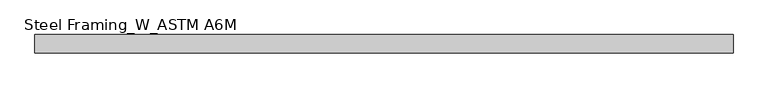
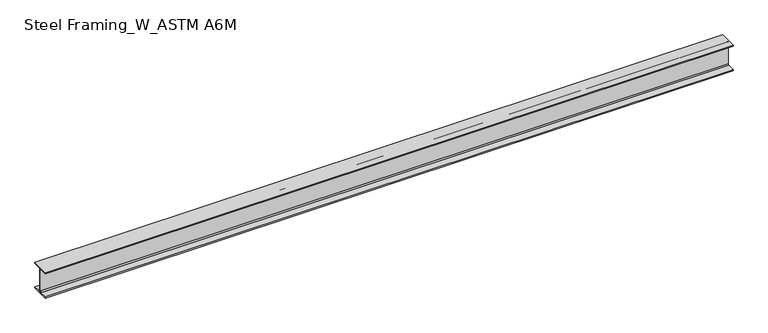
"""IFC4 building model written with IfcOpenShell, lengths in millimetres: beam geometry, Steel Framing_W_ASTM A6M : H_SB_AR_S02_W310x60_B5."""

import ifcopenshell
import ifcopenshell.guid

model = None  # the IFC model being written
_history = None  # IfcOwnerHistory: only IFC2X3 demands one
_inside = {}  # id of a spatial element -> (the spatial element, [elements in it])
_under = {}  # id of a project, library or spatial element -> (it, [spatial elements below it])
_declared = {}  # id of a project -> (the project, [libraries it declares])
_typed = {}  # id of a type object -> (the type object, [elements of that type])
_made_of = {}  # id of a material, layer set ... -> (it, [elements and type objects made of it])


def new_model(schema):
    """Start an empty IFC model of exactly this schema.

    Asked for "IFC4X3", IfcOpenShell would pick the latest addendum, in which some entities
    have other attributes; the version numbers below select the first issue.
    IFC2X3 requires an IfcOwnerHistory on every rooted entity: one is made here for all.
    """
    global model, _history
    if schema == "IFC4X3":
        model = ifcopenshell.file(schema_version=(4, 3, 0, 0))
    else:
        model = ifcopenshell.file(schema=schema)
    _inside.clear()
    _under.clear()
    _declared.clear()
    _typed.clear()
    _made_of.clear()
    _history = None
    if model.schema == "IFC2X3":
        org = make("IfcOrganization", Name="unknown")
        user = make(
            "IfcPersonAndOrganization",
            ThePerson=make("IfcPerson", FamilyName="unknown"),
            TheOrganization=org,
        )
        app = make(
            "IfcApplication",
            ApplicationDeveloper=org,
            Version="unknown",
            ApplicationFullName="unknown",
            ApplicationIdentifier="unknown",
        )
        _history = make(
            "IfcOwnerHistory",
            OwningUser=user,
            OwningApplication=app,
            ChangeAction="ADDED",
            CreationDate=0,
        )
    return model


def make(cls, **values):
    """One entity of the class cls with the attributes given. An attribute that is None is left unset."""
    return model.create_entity(
        cls, **{name: value for name, value in values.items() if value is not None}
    )


def rooted(cls, **values):
    """An entity with a GlobalId (a new one), such as an element, a storey or a relation."""
    return make(cls, GlobalId=ifcopenshell.guid.new(), OwnerHistory=_history, **values)


def si_unit(unit_type, name, prefix=None):
    """IfcSIUnit, for example si_unit("LENGTHUNIT", "METRE", prefix="MILLI")."""
    return make("IfcSIUnit", UnitType=unit_type, Prefix=prefix, Name=name)


def assignment(units):
    """IfcUnitAssignment: the units of a project."""
    return None if units is None else make("IfcUnitAssignment", Units=units)


def point(xyz):
    """IfcCartesianPoint."""
    return None if xyz is None else make("IfcCartesianPoint", Coordinates=xyz)


def direction(xyz):
    """IfcDirection."""
    return None if xyz is None else make("IfcDirection", DirectionRatios=xyz)


def frame(location, z_axis=None, x_axis=None):
    """IfcAxis2Placement3D, a coordinate frame: its origin and axes. An axis left out is left unset."""
    return make(
        "IfcAxis2Placement3D",
        Location=point(location),
        Axis=direction(z_axis),
        RefDirection=direction(x_axis),
    )


def frame_2d(location, x_axis=None):
    """IfcAxis2Placement2D, a coordinate frame in the plane: its origin and x axis."""
    return make(
        "IfcAxis2Placement2D", Location=point(location), RefDirection=direction(x_axis)
    )


def origin():
    """The frame at (0, 0, 0) with its axes left unset."""
    return frame((0.0, 0.0, 0.0))


def place(relative_to, where):
    """IfcLocalPlacement: puts the frame where relative to a parent placement (None: the world)."""
    return make(
        "IfcLocalPlacement", PlacementRelTo=relative_to, RelativePlacement=where
    )


def context(
    kind, dimensions, precision=None, world=None, true_north=None, identifier=None
):
    """IfcGeometricRepresentationContext, for example the 3D "Model" context."""
    return make(
        "IfcGeometricRepresentationContext",
        ContextIdentifier=identifier,
        ContextType=kind,
        CoordinateSpaceDimension=dimensions,
        Precision=precision,
        WorldCoordinateSystem=world,
        TrueNorth=true_north,
    )


def project(units=None, contexts=None):
    """IfcProject with its units and contexts."""
    return rooted(
        "IfcProject",
        Name="project",
        RepresentationContexts=contexts,
        UnitsInContext=assignment(units),
    )


def spatial(cls, under=None, at=None, **own):
    """A site, building, storey or space (cls), placed at a placement, below another one or the project."""
    s = rooted(cls, ObjectPlacement=at, **own)
    if under is not None:
        _under.setdefault(under.id(), (under, []))[1].append(s)
    return s


def polyline(points):
    """IfcPolyline through the points."""
    return make("IfcPolyline", Points=[point(p) for p in points])


def circle_curve(where, radius):
    """IfcCircle in the frame where."""
    return make("IfcCircle", Position=where, Radius=radius)


def trimmed(basis, trim1, trim2, sense, master):
    """IfcTrimmedCurve: the piece of a basis curve between two trims."""
    return make(
        "IfcTrimmedCurve",
        BasisCurve=basis,
        Trim1=trim1,
        Trim2=trim2,
        SenseAgreement=sense,
        MasterRepresentation=master,
    )


def segment(curve, same_sense, transition):
    """IfcCompositeCurveSegment."""
    return make(
        "IfcCompositeCurveSegment",
        Transition=transition,
        SameSense=same_sense,
        ParentCurve=curve,
    )


def composite_curve(segments, self_intersect=None):
    """IfcCompositeCurve: segments joined end to end."""
    return make("IfcCompositeCurve", Segments=segments, SelfIntersect=self_intersect)


def outline(outer, holes=None, kind="AREA"):
    """IfcArbitraryClosedProfileDef: a profile drawn as a closed curve; with holes, ...WithVoids."""
    if holes is None:
        return make("IfcArbitraryClosedProfileDef", ProfileType=kind, OuterCurve=outer)
    return make(
        "IfcArbitraryProfileDefWithVoids",
        ProfileType=kind,
        OuterCurve=outer,
        InnerCurves=holes,
    )


def extrude(swept, where, along, depth):
    """IfcExtrudedAreaSolid: the profile swept, set in the frame where, extruded along a direction by depth."""
    return make(
        "IfcExtrudedAreaSolid",
        SweptArea=swept,
        Position=where,
        ExtrudedDirection=direction(along),
        Depth=depth,
    )


def shape(context_of_items, identifier, shape_type, items):
    """IfcShapeRepresentation: the items that make up one representation, for example the "Body"."""
    return make(
        "IfcShapeRepresentation",
        ContextOfItems=context_of_items,
        RepresentationIdentifier=identifier,
        RepresentationType=shape_type,
        Items=items,
    )


def source(mapping_origin, context_of_items, identifier, shape_type, items):
    """IfcRepresentationMap: a shape defined once, which mapped items show again and again."""
    return make(
        "IfcRepresentationMap",
        MappingOrigin=mapping_origin,
        MappedRepresentation=shape(context_of_items, identifier, shape_type, items),
    )


def transform(
    local_origin,
    x_axis=None,
    y_axis=None,
    z_axis=None,
    scale=None,
    scale2=None,
    scale3=None,
    uniform=True,
):
    """IfcCartesianTransformationOperator3D, or its non-uniform kind. x_axis, y_axis, z_axis: its Axis1, 2, 3."""
    if uniform:
        return make(
            "IfcCartesianTransformationOperator3D",
            Axis1=direction(x_axis),
            Axis2=direction(y_axis),
            LocalOrigin=point(local_origin),
            Scale=scale,
            Axis3=direction(z_axis),
        )
    return make(
        "IfcCartesianTransformationOperator3DnonUniform",
        Axis1=direction(x_axis),
        Axis2=direction(y_axis),
        LocalOrigin=point(local_origin),
        Scale=scale,
        Axis3=direction(z_axis),
        Scale2=scale2,
        Scale3=scale3,
    )


def mapped(mapping_source, mapping_target):
    """IfcMappedItem: shows the shape of a source again, moved by a transform."""
    return make(
        "IfcMappedItem", MappingSource=mapping_source, MappingTarget=mapping_target
    )


def made_of(thing, what):
    """Note that an element or type object is made of a material, layer set ...; save() writes the relation."""
    if what is not None:
        _made_of.setdefault(what.id(), (what, []))[1].append(thing)
    return thing


def element(
    cls,
    number,
    at=None,
    inside=None,
    cuts=None,
    type_object=None,
    material=None,
    context=None,
    identifier="Body",
    shape_type=None,
    held_by="IfcProductDefinitionShape",
    body=None,
    shapes=None,
    **own,
):
    """One element of the class cls, such as IfcWall. Its Tag is "e" and its number.

    at: its placement. inside: the storey or other place that contains it. cuts: it is an
    opening in that element (IfcRelVoidsElement). A single representation is given by context,
    identifier, shape_type and body (its items); several are given by shapes. held_by: the class
    of the entity that holds the representations. save() writes the other relations.
    """
    e = rooted(cls, Tag="e%d" % number, ObjectPlacement=at, **own)
    if body is not None:
        shapes = [shape(context, identifier, shape_type, body)]
    if shapes is not None:
        e.Representation = make(held_by, Representations=shapes)
    if inside is not None:
        _inside.setdefault(inside.id(), (inside, []))[1].append(e)
    if cuts is not None:
        rooted(
            "IfcRelVoidsElement", RelatingBuildingElement=cuts, RelatedOpeningElement=e
        )
    if type_object is not None:
        _typed.setdefault(type_object.id(), (type_object, []))[1].append(e)
    return made_of(e, material)


def aggregate(whole, parts):
    """IfcRelAggregates: a whole, such as a stair, and the parts it consists of."""
    return rooted("IfcRelAggregates", RelatingObject=whole, RelatedObjects=parts)


def save(model, path):
    """Write the relations noted so far, then the file.

    IfcRelAggregates (storeys below a building ...), IfcRelContainedInSpatialStructure (elements
    in a storey), IfcRelDefinesByType, IfcRelAssociatesMaterial and IfcRelDeclares: one each for
    every whole, place, type object, material and project.
    """
    for whole, parts in _under.values():
        aggregate(whole, parts)
    for where, things in _inside.values():
        rooted(
            "IfcRelContainedInSpatialStructure",
            RelatedElements=things,
            RelatingStructure=where,
        )
    for kind, things in _typed.values():
        rooted("IfcRelDefinesByType", RelatedObjects=things, RelatingType=kind)
    for what, things in _made_of.values():
        rooted("IfcRelAssociatesMaterial", RelatedObjects=things, RelatingMaterial=what)
    for by, libraries in _declared.values():
        rooted("IfcRelDeclares", RelatingContext=by, RelatedDefinitions=libraries)
    model.write(path)


def steel_framing_w_astm_a6m_97b597d5(model_context):
    return source(origin(), model_context, "Body", "SweptSolid", [
        extrude(outline(composite_curve([segment(polyline([(101.5, -137.9), (101.5, -151.0), (-101.5, -151.0), (-101.5, -137.9), (-16.545, -137.9)]), True, "CONTINUOUS"), segment(trimmed(circle_curve(frame_2d((-16.545, -125.1)), 12.8), [point((-16.545, -137.9))], [point((-3.745, -125.1))], True, "CARTESIAN"), True, "CONTINUOUS"), segment(polyline([(-3.745, -125.1), (-3.745, 125.1)]), True, "CONTINUOUS"), segment(trimmed(circle_curve(frame_2d((-16.545, 125.1)), 12.8), [point((-3.745, 125.1))], [point((-16.545, 137.9))], True, "CARTESIAN"), True, "CONTINUOUS"), segment(polyline([(-16.545, 137.9), (-101.5, 137.9), (-101.5, 151.0), (101.5, 151.0), (101.5, 137.9), (16.545, 137.9)]), True, "CONTINUOUS"), segment(trimmed(circle_curve(frame_2d((16.545, 125.1)), 12.8), [point((16.545, 137.9))], [point((3.745, 125.1))], True, "CARTESIAN"), True, "CONTINUOUS"), segment(polyline([(3.745, 125.1), (3.745, -125.1)]), True, "CONTINUOUS"), segment(trimmed(circle_curve(frame_2d((16.545, -125.1)), 12.8), [point((3.745, -125.1))], [point((16.545, -137.9))], True, "CARTESIAN"), True, "CONTINUOUS"), segment(polyline([(16.545, -137.9), (101.5, -137.9)]), True, "CONTINUOUS")], self_intersect=False)), frame((-3884.3, 0.0, 0.0), z_axis=(1.0, 0.0, 0.0), x_axis=(0.0, 1.0, 0.0)), (0.0, 0.0, 1.0), 7698.8),
    ])


if __name__ == "__main__":
    model = new_model("IFC4")
    model_context = context("Model", 3, world=origin())
    ifc_project = project(units=[si_unit("LENGTHUNIT", "METRE", prefix="MILLI")], contexts=[model_context])
    site = spatial("IfcSite", under=ifc_project)
    building = spatial("IfcBuilding", under=site)
    placement = place(None, origin())
    steel_framing_w_astm_a6m_shape = steel_framing_w_astm_a6m_97b597d5(model_context)
    element("IfcBeam", 1, ObjectType="Steel Framing_W_ASTM A6M : H_SB_AR_S02_W310x60_B5", at=placement, inside=building, context=model_context, shape_type="MappedRepresentation", body=[
        mapped(steel_framing_w_astm_a6m_shape, transform((0.0, 0.0, 0.0), x_axis=(1.0, 0.0, 0.0), y_axis=(0.0, 1.0, 0.0), z_axis=(0.0, 0.0, 1.0))),
    ])
    save(model, "model.ifc")

# Revit data of these elements
# Type "Steel Framing_W_ASTM A6M : H_SB_AR_S02_W310x60_B5"
#   Type Mark = "B5"
#   Section Name Key = "W12x40"
#   Width = 20.3 cm
#   Web Thickness = 0.749 cm
#   Web Fillet = 1.28 cm
#   Warping Constant = 387000.0 cm⁶
#   Torsional Moment of Inertia = 37.70 cm⁴
#   Section Area = 75.5 cm²
#   Plastic Modulus weak axis = 275.0 cm³
#   Plastic Modulus strong axis = 934.0 cm³
#   Perimeter = 1.38 m²/m
#   Nominal Weight = 60.00 kgf/m
#   Moment of Inertia weak axis = 1840.00 cm⁴
#   Moment of Inertia strong axis = 12800.00 cm⁴
#   Height = 30.2 cm
#   Flange Thickness = 1.31 cm
#   Elastic Modulus weak axis = 180.0 cm³
#   Elastic Modulus strong axis = 844.0 cm³
#   Centroid Vertical = 15.1 cm
#   Centroid Horizontal = 10.15 cm
#   Length [instance default] = 1500 mm
#   Structural Material [instance default] = Steel, 45-345
#   Bolt Spacing = 0
#   Assembly Code = ""
# Element 1 (IfcBeam, "Steel Framing_W_ASTM A6M : H_SB_AR_S02_W310x60_B5")
#   Materials on its faces: "Steel, 45-345"
# Materials
#   "Steel, 45-345": class "Metal", colour RGB 189 187 185, transparency 0, Description = "Steel 345 MPa", Cost = 0
